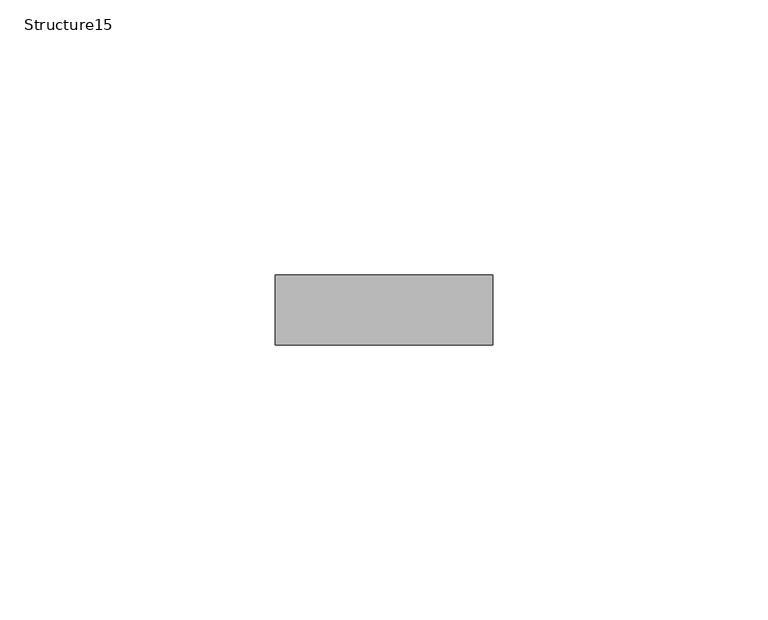
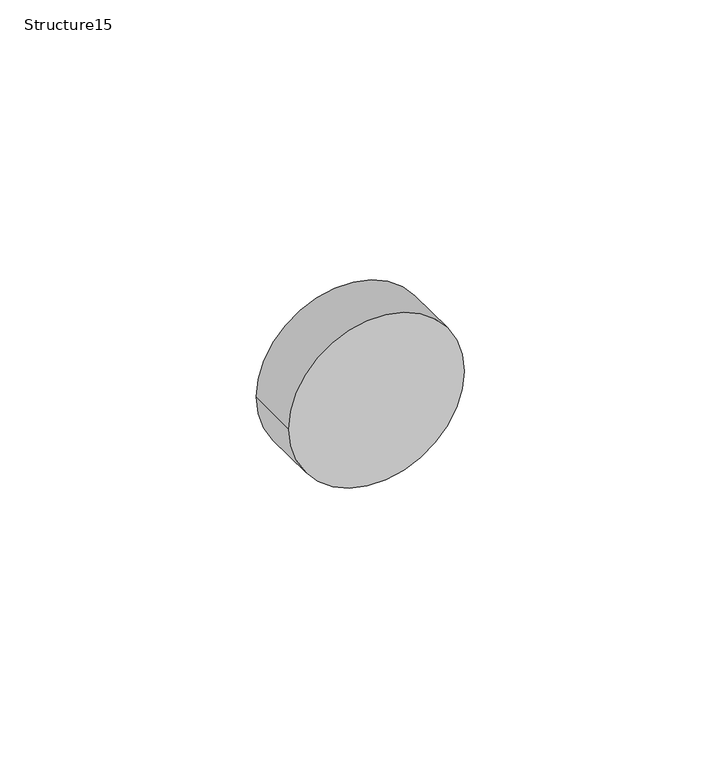
"""IFC4 building model written with IfcOpenShell, lengths in millimetres: proxy geometry, Structure15 : Structure668217136."""

from ifc_helpers import new_model, si_unit, point, frame, frame_2d, origin, place, context, project, spatial, circle_curve, trimmed, segment, composite_curve, outline, extrude, source, transform, mapped, element, save


def structure15_8c04c62a(model_context):
    return source(origin(), model_context, "Body", "SweptSolid", [
        extrude(outline(composite_curve([segment(trimmed(circle_curve(frame_2d((38047.8454063, 5185.7383658)), 19.7708678), [point((38047.8454063, 5165.967498))], [point((38047.8454063, 5205.5092336))], False, "CARTESIAN"), True, "CONTINUOUS"), segment(trimmed(circle_curve(frame_2d((38047.8454063, 5185.7383658)), 19.7708678), [point((38047.8454063, 5205.5092336))], [point((38047.8454063, 5165.967498))], False, "CARTESIAN"), True, "CONTINUOUS")], self_intersect=False)), frame((0.0, 1964.2572934, 0.0), z_axis=(0.0, 1.0, 0.0), x_axis=(0.0, 0.0, 1.0)), (0.0, 0.0, 1.0), 12.7),
    ])


if __name__ == "__main__":
    model = new_model("IFC4")
    model_context = context("Model", 3, world=origin())
    ifc_project = project(units=[si_unit("LENGTHUNIT", "METRE", prefix="MILLI")], contexts=[model_context])
    site = spatial("IfcSite", under=ifc_project)
    building = spatial("IfcBuilding", under=site)
    placement = place(None, origin())
    structure15_shape = structure15_8c04c62a(model_context)
    element("IfcBuildingElementProxy", 1, Name="Structure15 : Structure668217136", ObjectType="Structure15 : Structure668217136", at=placement, inside=building, context=model_context, shape_type="MappedRepresentation", body=[
        mapped(structure15_shape, transform((0.0, 0.0, 0.0), x_axis=(1.0, 0.0, 0.0), y_axis=(0.0, 1.0, 0.0), z_axis=(0.0, 0.0, 1.0))),
    ])
    save(model, "model.ifc")

# Revit data of these elements
# Type "Structure15 : Structure668217136"
#   NameOverride = "Structure668217136"
# Element 1 (IfcBuildingElementProxy, "Structure15 : Structure668217136")
#   Materials on its faces: "1.5\" DIA. STAINLESS STEEL RAILING"
# Materials
#   "1.5\" DIA. STAINLESS STEEL RAILING": class "Unassigned", colour RGB 128 128 128, transparency 0, Cost = 0
